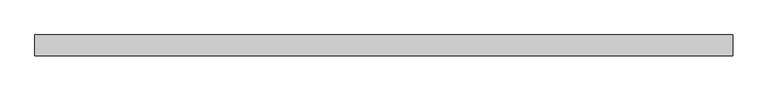
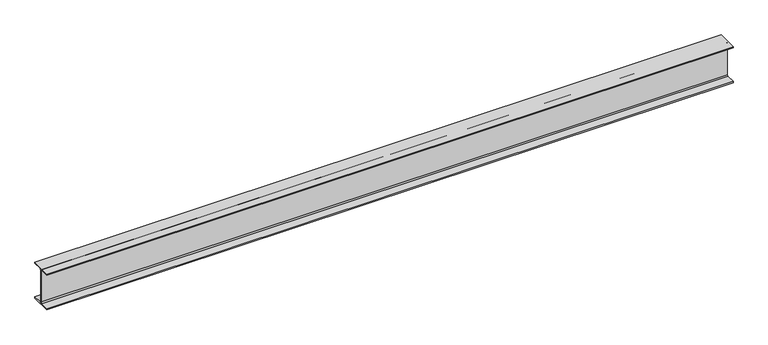
"""IFC4 building model written with IfcOpenShell, lengths in millimetres: beam geometry, Old_Steel Beam_H-KSD3502 : H_SB_ASB_H-482×300x11x15."""

from ifc_helpers import new_model, si_unit, point, frame, frame_2d, origin, place, context, project, spatial, polyline, circle_curve, trimmed, segment, composite_curve, outline, extrude, source, transform, mapped, element, save


def beam_5b57ae8e(model_context):
    return source(origin(), model_context, "Body", "SweptSolid", [
        extrude(outline(composite_curve([segment(polyline([(82.5, -141.5), (82.5, -151.7), (-82.5, -151.7), (-82.5, -141.5), (-11.9, -141.5)]), True, "CONTINUOUS"), segment(trimmed(circle_curve(frame_2d((-11.9, -132.6)), 8.9), [point((-11.9, -141.5))], [point((-3.0, -132.6))], True, "CARTESIAN"), True, "CONTINUOUS"), segment(polyline([(-3.0, -132.6), (-3.0, 132.6)]), True, "CONTINUOUS"), segment(trimmed(circle_curve(frame_2d((-11.9, 132.6)), 8.9), [point((-3.0, 132.6))], [point((-11.9, 141.5))], True, "CARTESIAN"), True, "CONTINUOUS"), segment(polyline([(-11.9, 141.5), (-82.5, 141.5), (-82.5, 151.7), (82.5, 151.7), (82.5, 141.5), (11.9, 141.5)]), True, "CONTINUOUS"), segment(trimmed(circle_curve(frame_2d((11.9, 132.6)), 8.9), [point((11.9, 141.5))], [point((3.0, 132.6))], True, "CARTESIAN"), True, "CONTINUOUS"), segment(polyline([(3.0, 132.6), (3.0, -132.6)]), True, "CONTINUOUS"), segment(trimmed(circle_curve(frame_2d((11.9, -132.6)), 8.9), [point((3.0, -132.6))], [point((11.9, -141.5))], True, "CARTESIAN"), True, "CONTINUOUS"), segment(polyline([(11.9, -141.5), (82.5, -141.5)]), True, "CONTINUOUS")], self_intersect=False)), frame((-2662.3, 0.0, 0.0), z_axis=(1.0, 0.0, 0.0), x_axis=(0.0, 1.0, 0.0)), (0.0, 0.0, 1.0), 5487.3),
    ])


if __name__ == "__main__":
    model = new_model("IFC4")
    model_context = context("Model", 3, world=origin())
    ifc_project = project(units=[si_unit("LENGTHUNIT", "METRE", prefix="MILLI")], contexts=[model_context])
    site = spatial("IfcSite", under=ifc_project)
    building = spatial("IfcBuilding", under=site)
    placement = place(None, origin())
    beam_shape = beam_5b57ae8e(model_context)
    element("IfcBeam", 1, ObjectType="Old_Steel Beam_H-KSD3502 : H_SB_ASB_H-482×300x11x15", at=placement, inside=building, context=model_context, shape_type="MappedRepresentation", body=[
        mapped(beam_shape, transform((0.0, 0.0, 0.0), x_axis=(1.0, 0.0, 0.0), y_axis=(0.0, 1.0, 0.0), z_axis=(0.0, 0.0, 1.0))),
    ])
    save(model, "model.ifc")

# Revit data of these elements
# Type "Old_Steel Beam_H-KSD3502 : H_SB_ASB_H-482×300x11x15"
#   Width = 30.0 cm
#   Web Thickness = 1.1 cm
#   Web Fillet = 2.6 cm
#   Warping Constant = 3680250.0 cm⁶
#   Torsional Moment of Inertia = 88.2192 cm⁴
#   Torsional Modulus = 1.0 cm³
#   Section Area = 145.5 cm²
#   Plastic Modulus weak axis = 695.0 cm³
#   Plastic Modulus strong axis = 2790.0 cm³
#   Perimeter = 2.10 m²/m
#   Nominal Weight = 114.00 kgf/m
#   Moment of Inertia weak axis = 6760.00 cm⁴
#   Moment of Inertia strong axis = 60400.00 cm⁴
#   Height = 48.2 cm
#   Flange Thickness = 1.5 cm
#   Elastic Modulus weak axis = 451.0 cm³
#   Elastic Modulus strong axis = 2500.0 cm³
#   Centroid Vertical = 24.1 cm
#   Centroid Horizontal = 15.0 cm
#   Length [instance default] = 1.5240 m
#   Structural Material [instance default] = Steel, 45-345
#   Assembly Code = ""
# Element 1 (IfcBeam, "Old_Steel Beam_H-KSD3502 : H_SB_ASB_H-482×300x11x15")
#   Structural Material = none
# Materials
#   "Steel, 45-345": class "Metal", colour RGB 189 187 185, transparency 0, Description = "Steel 345 MPa", Cost = 0
